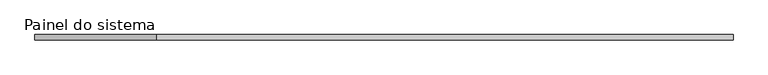
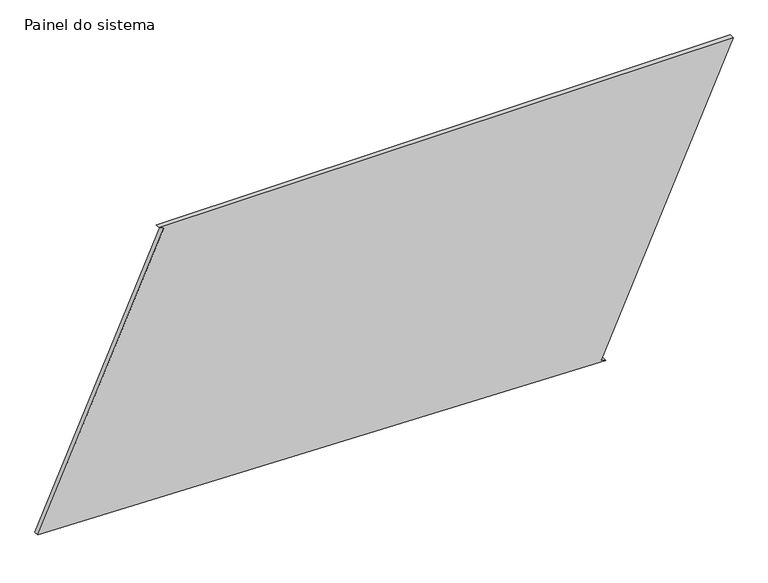
"""IFC4 building model written with IfcOpenShell, lengths in millimetres: plate geometry, Painel do sistema : Envidraçado."""

import ifcopenshell
import ifcopenshell.guid

model = None  # the IFC model being written
_history = None  # IfcOwnerHistory: only IFC2X3 demands one
_inside = {}  # id of a spatial element -> (the spatial element, [elements in it])
_under = {}  # id of a project, library or spatial element -> (it, [spatial elements below it])
_declared = {}  # id of a project -> (the project, [libraries it declares])
_typed = {}  # id of a type object -> (the type object, [elements of that type])
_made_of = {}  # id of a material, layer set ... -> (it, [elements and type objects made of it])


def new_model(schema):
    """Start an empty IFC model of exactly this schema.

    Asked for "IFC4X3", IfcOpenShell would pick the latest addendum, in which some entities
    have other attributes; the version numbers below select the first issue.
    IFC2X3 requires an IfcOwnerHistory on every rooted entity: one is made here for all.
    """
    global model, _history
    if schema == "IFC4X3":
        model = ifcopenshell.file(schema_version=(4, 3, 0, 0))
    else:
        model = ifcopenshell.file(schema=schema)
    _inside.clear()
    _under.clear()
    _declared.clear()
    _typed.clear()
    _made_of.clear()
    _history = None
    if model.schema == "IFC2X3":
        org = make("IfcOrganization", Name="unknown")
        user = make(
            "IfcPersonAndOrganization",
            ThePerson=make("IfcPerson", FamilyName="unknown"),
            TheOrganization=org,
        )
        app = make(
            "IfcApplication",
            ApplicationDeveloper=org,
            Version="unknown",
            ApplicationFullName="unknown",
            ApplicationIdentifier="unknown",
        )
        _history = make(
            "IfcOwnerHistory",
            OwningUser=user,
            OwningApplication=app,
            ChangeAction="ADDED",
            CreationDate=0,
        )
    return model


def make(cls, **values):
    """One entity of the class cls with the attributes given. An attribute that is None is left unset."""
    return model.create_entity(
        cls, **{name: value for name, value in values.items() if value is not None}
    )


def rooted(cls, **values):
    """An entity with a GlobalId (a new one), such as an element, a storey or a relation."""
    return make(cls, GlobalId=ifcopenshell.guid.new(), OwnerHistory=_history, **values)


def si_unit(unit_type, name, prefix=None):
    """IfcSIUnit, for example si_unit("LENGTHUNIT", "METRE", prefix="MILLI")."""
    return make("IfcSIUnit", UnitType=unit_type, Prefix=prefix, Name=name)


def assignment(units):
    """IfcUnitAssignment: the units of a project."""
    return None if units is None else make("IfcUnitAssignment", Units=units)


def point(xyz):
    """IfcCartesianPoint."""
    return None if xyz is None else make("IfcCartesianPoint", Coordinates=xyz)


def direction(xyz):
    """IfcDirection."""
    return None if xyz is None else make("IfcDirection", DirectionRatios=xyz)


def frame(location, z_axis=None, x_axis=None):
    """IfcAxis2Placement3D, a coordinate frame: its origin and axes. An axis left out is left unset."""
    return make(
        "IfcAxis2Placement3D",
        Location=point(location),
        Axis=direction(z_axis),
        RefDirection=direction(x_axis),
    )


def origin():
    """The frame at (0, 0, 0) with its axes left unset."""
    return frame((0.0, 0.0, 0.0))


def place(relative_to, where):
    """IfcLocalPlacement: puts the frame where relative to a parent placement (None: the world)."""
    return make(
        "IfcLocalPlacement", PlacementRelTo=relative_to, RelativePlacement=where
    )


def context(
    kind, dimensions, precision=None, world=None, true_north=None, identifier=None
):
    """IfcGeometricRepresentationContext, for example the 3D "Model" context."""
    return make(
        "IfcGeometricRepresentationContext",
        ContextIdentifier=identifier,
        ContextType=kind,
        CoordinateSpaceDimension=dimensions,
        Precision=precision,
        WorldCoordinateSystem=world,
        TrueNorth=true_north,
    )


def project(units=None, contexts=None):
    """IfcProject with its units and contexts."""
    return rooted(
        "IfcProject",
        Name="project",
        RepresentationContexts=contexts,
        UnitsInContext=assignment(units),
    )


def spatial(cls, under=None, at=None, **own):
    """A site, building, storey or space (cls), placed at a placement, below another one or the project."""
    s = rooted(cls, ObjectPlacement=at, **own)
    if under is not None:
        _under.setdefault(under.id(), (under, []))[1].append(s)
    return s


def polyline(points):
    """IfcPolyline through the points."""
    return make("IfcPolyline", Points=[point(p) for p in points])


def outline(outer, holes=None, kind="AREA"):
    """IfcArbitraryClosedProfileDef: a profile drawn as a closed curve; with holes, ...WithVoids."""
    if holes is None:
        return make("IfcArbitraryClosedProfileDef", ProfileType=kind, OuterCurve=outer)
    return make(
        "IfcArbitraryProfileDefWithVoids",
        ProfileType=kind,
        OuterCurve=outer,
        InnerCurves=holes,
    )


def extrude(swept, where, along, depth):
    """IfcExtrudedAreaSolid: the profile swept, set in the frame where, extruded along a direction by depth."""
    return make(
        "IfcExtrudedAreaSolid",
        SweptArea=swept,
        Position=where,
        ExtrudedDirection=direction(along),
        Depth=depth,
    )


def shape(context_of_items, identifier, shape_type, items):
    """IfcShapeRepresentation: the items that make up one representation, for example the "Body"."""
    return make(
        "IfcShapeRepresentation",
        ContextOfItems=context_of_items,
        RepresentationIdentifier=identifier,
        RepresentationType=shape_type,
        Items=items,
    )


def source(mapping_origin, context_of_items, identifier, shape_type, items):
    """IfcRepresentationMap: a shape defined once, which mapped items show again and again."""
    return make(
        "IfcRepresentationMap",
        MappingOrigin=mapping_origin,
        MappedRepresentation=shape(context_of_items, identifier, shape_type, items),
    )


def transform(
    local_origin,
    x_axis=None,
    y_axis=None,
    z_axis=None,
    scale=None,
    scale2=None,
    scale3=None,
    uniform=True,
):
    """IfcCartesianTransformationOperator3D, or its non-uniform kind. x_axis, y_axis, z_axis: its Axis1, 2, 3."""
    if uniform:
        return make(
            "IfcCartesianTransformationOperator3D",
            Axis1=direction(x_axis),
            Axis2=direction(y_axis),
            LocalOrigin=point(local_origin),
            Scale=scale,
            Axis3=direction(z_axis),
        )
    return make(
        "IfcCartesianTransformationOperator3DnonUniform",
        Axis1=direction(x_axis),
        Axis2=direction(y_axis),
        LocalOrigin=point(local_origin),
        Scale=scale,
        Axis3=direction(z_axis),
        Scale2=scale2,
        Scale3=scale3,
    )


def mapped(mapping_source, mapping_target):
    """IfcMappedItem: shows the shape of a source again, moved by a transform."""
    return make(
        "IfcMappedItem", MappingSource=mapping_source, MappingTarget=mapping_target
    )


def made_of(thing, what):
    """Note that an element or type object is made of a material, layer set ...; save() writes the relation."""
    if what is not None:
        _made_of.setdefault(what.id(), (what, []))[1].append(thing)
    return thing


def element(
    cls,
    number,
    at=None,
    inside=None,
    cuts=None,
    type_object=None,
    material=None,
    context=None,
    identifier="Body",
    shape_type=None,
    held_by="IfcProductDefinitionShape",
    body=None,
    shapes=None,
    **own,
):
    """One element of the class cls, such as IfcWall. Its Tag is "e" and its number.

    at: its placement. inside: the storey or other place that contains it. cuts: it is an
    opening in that element (IfcRelVoidsElement). A single representation is given by context,
    identifier, shape_type and body (its items); several are given by shapes. held_by: the class
    of the entity that holds the representations. save() writes the other relations.
    """
    e = rooted(cls, Tag="e%d" % number, ObjectPlacement=at, **own)
    if body is not None:
        shapes = [shape(context, identifier, shape_type, body)]
    if shapes is not None:
        e.Representation = make(held_by, Representations=shapes)
    if inside is not None:
        _inside.setdefault(inside.id(), (inside, []))[1].append(e)
    if cuts is not None:
        rooted(
            "IfcRelVoidsElement", RelatingBuildingElement=cuts, RelatedOpeningElement=e
        )
    if type_object is not None:
        _typed.setdefault(type_object.id(), (type_object, []))[1].append(e)
    return made_of(e, material)


def aggregate(whole, parts):
    """IfcRelAggregates: a whole, such as a stair, and the parts it consists of."""
    return rooted("IfcRelAggregates", RelatingObject=whole, RelatedObjects=parts)


def save(model, path):
    """Write the relations noted so far, then the file.

    IfcRelAggregates (storeys below a building ...), IfcRelContainedInSpatialStructure (elements
    in a storey), IfcRelDefinesByType, IfcRelAssociatesMaterial and IfcRelDeclares: one each for
    every whole, place, type object, material and project.
    """
    for whole, parts in _under.values():
        aggregate(whole, parts)
    for where, things in _inside.values():
        rooted(
            "IfcRelContainedInSpatialStructure",
            RelatedElements=things,
            RelatingStructure=where,
        )
    for kind, things in _typed.values():
        rooted("IfcRelDefinesByType", RelatedObjects=things, RelatingType=kind)
    for what, things in _made_of.values():
        rooted("IfcRelAssociatesMaterial", RelatedObjects=things, RelatingMaterial=what)
    for by, libraries in _declared.values():
        rooted("IfcRelDeclares", RelatingContext=by, RelatedDefinitions=libraries)
    model.write(path)


def painel_do_sistema_fb3da87d(model_context):
    return source(origin(), model_context, "Body", "SweptSolid", [
        extrude(outline(polyline([(0.0, 1071.2864505), (10.2299965, 1048.475331), (1442.2393746, 1690.6819101), (1442.2393746, -1101.4091832), (1432.0093781, -1078.5980637), (67.1684736, -1690.6819101), (0.0, 1071.2864505)])), frame((0.0, 24.5, 0.0), z_axis=(0.0, 1.0, 0.0), x_axis=(0.0, 0.0, 1.0)), (0.0, 0.0, 1.0), 25.0),
    ])


if __name__ == "__main__":
    model = new_model("IFC4")
    model_context = context("Model", 3, world=origin())
    ifc_project = project(units=[si_unit("LENGTHUNIT", "METRE", prefix="MILLI")], contexts=[model_context])
    site = spatial("IfcSite", under=ifc_project)
    building = spatial("IfcBuilding", under=site)
    placement = place(None, origin())
    painel_do_sistema_shape = painel_do_sistema_fb3da87d(model_context)
    element("IfcPlate", 1, ObjectType="Painel do sistema : Envidraçado", at=placement, inside=building, context=model_context, shape_type="MappedRepresentation", body=[
        mapped(painel_do_sistema_shape, transform((0.0, 0.0, 0.0), x_axis=(1.0, 0.0, 0.0), y_axis=(0.0, 1.0, 0.0), z_axis=(0.0, 0.0, 1.0))),
    ])
    save(model, "model.ifc")

# Revit data of these elements
# Type "Painel do sistema : Envidraçado"
#   Construction Type Id = "GSP4R"
#   Analytic Construction = "Vidraça única Pilkington 1/8 pol"
#   Visual Light Transmittance = 0.9
#   Solar Heat Gain Coefficient = 0.86
#   Heat Transfer Coefficient (U) = 6.7069 W/(m²·K)
# Element 1 (IfcPlate, "Painel do sistema : Envidraçado")
#   Materials on its faces: "Vidro"
# Materials
#   "Vidro": class "Vidro", colour RGB 0 128 192, transparency 0.9, Description = "Vidro de sílica", Cost = 0
